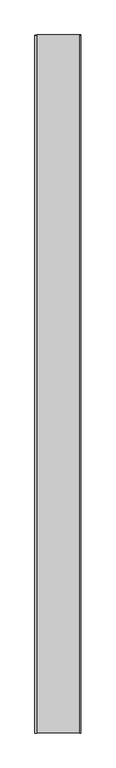
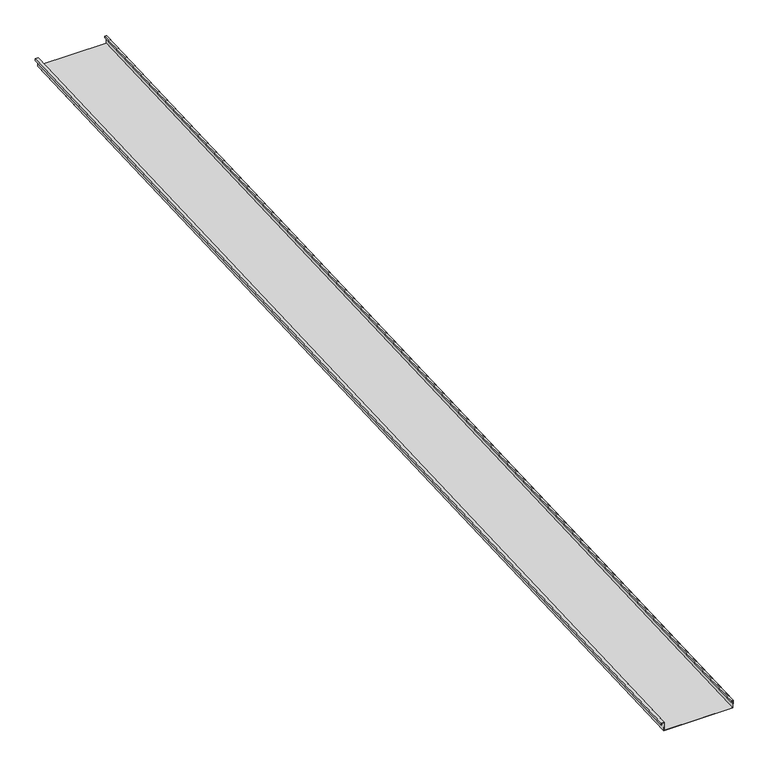
"""IFC4 building model written with IfcOpenShell, lengths in millimetres: proxy geometry, Generic Models 2:Generic Models 2:310765:Generic Models 2:310765 : Generic Models 2:Generic Models 2:310765:103 : Generic Models 2:Generic Models 2:310765:Generic Models 2:310765 : Generic Models 2:Generic Models 2:310765:300385."""

import ifcopenshell
import ifcopenshell.guid

model = None  # the IFC model being written
_history = None  # IfcOwnerHistory: only IFC2X3 demands one
_inside = {}  # id of a spatial element -> (the spatial element, [elements in it])
_under = {}  # id of a project, library or spatial element -> (it, [spatial elements below it])
_declared = {}  # id of a project -> (the project, [libraries it declares])
_typed = {}  # id of a type object -> (the type object, [elements of that type])
_made_of = {}  # id of a material, layer set ... -> (it, [elements and type objects made of it])


def new_model(schema):
    """Start an empty IFC model of exactly this schema.

    Asked for "IFC4X3", IfcOpenShell would pick the latest addendum, in which some entities
    have other attributes; the version numbers below select the first issue.
    IFC2X3 requires an IfcOwnerHistory on every rooted entity: one is made here for all.
    """
    global model, _history
    if schema == "IFC4X3":
        model = ifcopenshell.file(schema_version=(4, 3, 0, 0))
    else:
        model = ifcopenshell.file(schema=schema)
    _inside.clear()
    _under.clear()
    _declared.clear()
    _typed.clear()
    _made_of.clear()
    _history = None
    if model.schema == "IFC2X3":
        org = make("IfcOrganization", Name="unknown")
        user = make(
            "IfcPersonAndOrganization",
            ThePerson=make("IfcPerson", FamilyName="unknown"),
            TheOrganization=org,
        )
        app = make(
            "IfcApplication",
            ApplicationDeveloper=org,
            Version="unknown",
            ApplicationFullName="unknown",
            ApplicationIdentifier="unknown",
        )
        _history = make(
            "IfcOwnerHistory",
            OwningUser=user,
            OwningApplication=app,
            ChangeAction="ADDED",
            CreationDate=0,
        )
    return model


def make(cls, **values):
    """One entity of the class cls with the attributes given. An attribute that is None is left unset."""
    return model.create_entity(
        cls, **{name: value for name, value in values.items() if value is not None}
    )


def rooted(cls, **values):
    """An entity with a GlobalId (a new one), such as an element, a storey or a relation."""
    return make(cls, GlobalId=ifcopenshell.guid.new(), OwnerHistory=_history, **values)


def si_unit(unit_type, name, prefix=None):
    """IfcSIUnit, for example si_unit("LENGTHUNIT", "METRE", prefix="MILLI")."""
    return make("IfcSIUnit", UnitType=unit_type, Prefix=prefix, Name=name)


def assignment(units):
    """IfcUnitAssignment: the units of a project."""
    return None if units is None else make("IfcUnitAssignment", Units=units)


def point(xyz):
    """IfcCartesianPoint."""
    return None if xyz is None else make("IfcCartesianPoint", Coordinates=xyz)


def direction(xyz):
    """IfcDirection."""
    return None if xyz is None else make("IfcDirection", DirectionRatios=xyz)


def frame(location, z_axis=None, x_axis=None):
    """IfcAxis2Placement3D, a coordinate frame: its origin and axes. An axis left out is left unset."""
    return make(
        "IfcAxis2Placement3D",
        Location=point(location),
        Axis=direction(z_axis),
        RefDirection=direction(x_axis),
    )


def origin():
    """The frame at (0, 0, 0) with its axes left unset."""
    return frame((0.0, 0.0, 0.0))


def place(relative_to, where):
    """IfcLocalPlacement: puts the frame where relative to a parent placement (None: the world)."""
    return make(
        "IfcLocalPlacement", PlacementRelTo=relative_to, RelativePlacement=where
    )


def context(
    kind, dimensions, precision=None, world=None, true_north=None, identifier=None
):
    """IfcGeometricRepresentationContext, for example the 3D "Model" context."""
    return make(
        "IfcGeometricRepresentationContext",
        ContextIdentifier=identifier,
        ContextType=kind,
        CoordinateSpaceDimension=dimensions,
        Precision=precision,
        WorldCoordinateSystem=world,
        TrueNorth=true_north,
    )


def project(units=None, contexts=None):
    """IfcProject with its units and contexts."""
    return rooted(
        "IfcProject",
        Name="project",
        RepresentationContexts=contexts,
        UnitsInContext=assignment(units),
    )


def spatial(cls, under=None, at=None, **own):
    """A site, building, storey or space (cls), placed at a placement, below another one or the project."""
    s = rooted(cls, ObjectPlacement=at, **own)
    if under is not None:
        _under.setdefault(under.id(), (under, []))[1].append(s)
    return s


def polyline(points):
    """IfcPolyline through the points."""
    return make("IfcPolyline", Points=[point(p) for p in points])


def outline(outer, holes=None, kind="AREA"):
    """IfcArbitraryClosedProfileDef: a profile drawn as a closed curve; with holes, ...WithVoids."""
    if holes is None:
        return make("IfcArbitraryClosedProfileDef", ProfileType=kind, OuterCurve=outer)
    return make(
        "IfcArbitraryProfileDefWithVoids",
        ProfileType=kind,
        OuterCurve=outer,
        InnerCurves=holes,
    )


def extrude(swept, where, along, depth):
    """IfcExtrudedAreaSolid: the profile swept, set in the frame where, extruded along a direction by depth."""
    return make(
        "IfcExtrudedAreaSolid",
        SweptArea=swept,
        Position=where,
        ExtrudedDirection=direction(along),
        Depth=depth,
    )


def shape(context_of_items, identifier, shape_type, items):
    """IfcShapeRepresentation: the items that make up one representation, for example the "Body"."""
    return make(
        "IfcShapeRepresentation",
        ContextOfItems=context_of_items,
        RepresentationIdentifier=identifier,
        RepresentationType=shape_type,
        Items=items,
    )


def source(mapping_origin, context_of_items, identifier, shape_type, items):
    """IfcRepresentationMap: a shape defined once, which mapped items show again and again."""
    return make(
        "IfcRepresentationMap",
        MappingOrigin=mapping_origin,
        MappedRepresentation=shape(context_of_items, identifier, shape_type, items),
    )


def transform(
    local_origin,
    x_axis=None,
    y_axis=None,
    z_axis=None,
    scale=None,
    scale2=None,
    scale3=None,
    uniform=True,
):
    """IfcCartesianTransformationOperator3D, or its non-uniform kind. x_axis, y_axis, z_axis: its Axis1, 2, 3."""
    if uniform:
        return make(
            "IfcCartesianTransformationOperator3D",
            Axis1=direction(x_axis),
            Axis2=direction(y_axis),
            LocalOrigin=point(local_origin),
            Scale=scale,
            Axis3=direction(z_axis),
        )
    return make(
        "IfcCartesianTransformationOperator3DnonUniform",
        Axis1=direction(x_axis),
        Axis2=direction(y_axis),
        LocalOrigin=point(local_origin),
        Scale=scale,
        Axis3=direction(z_axis),
        Scale2=scale2,
        Scale3=scale3,
    )


def mapped(mapping_source, mapping_target):
    """IfcMappedItem: shows the shape of a source again, moved by a transform."""
    return make(
        "IfcMappedItem", MappingSource=mapping_source, MappingTarget=mapping_target
    )


def made_of(thing, what):
    """Note that an element or type object is made of a material, layer set ...; save() writes the relation."""
    if what is not None:
        _made_of.setdefault(what.id(), (what, []))[1].append(thing)
    return thing


def element(
    cls,
    number,
    at=None,
    inside=None,
    cuts=None,
    type_object=None,
    material=None,
    context=None,
    identifier="Body",
    shape_type=None,
    held_by="IfcProductDefinitionShape",
    body=None,
    shapes=None,
    **own,
):
    """One element of the class cls, such as IfcWall. Its Tag is "e" and its number.

    at: its placement. inside: the storey or other place that contains it. cuts: it is an
    opening in that element (IfcRelVoidsElement). A single representation is given by context,
    identifier, shape_type and body (its items); several are given by shapes. held_by: the class
    of the entity that holds the representations. save() writes the other relations.
    """
    e = rooted(cls, Tag="e%d" % number, ObjectPlacement=at, **own)
    if body is not None:
        shapes = [shape(context, identifier, shape_type, body)]
    if shapes is not None:
        e.Representation = make(held_by, Representations=shapes)
    if inside is not None:
        _inside.setdefault(inside.id(), (inside, []))[1].append(e)
    if cuts is not None:
        rooted(
            "IfcRelVoidsElement", RelatingBuildingElement=cuts, RelatedOpeningElement=e
        )
    if type_object is not None:
        _typed.setdefault(type_object.id(), (type_object, []))[1].append(e)
    return made_of(e, material)


def aggregate(whole, parts):
    """IfcRelAggregates: a whole, such as a stair, and the parts it consists of."""
    return rooted("IfcRelAggregates", RelatingObject=whole, RelatedObjects=parts)


def save(model, path):
    """Write the relations noted so far, then the file.

    IfcRelAggregates (storeys below a building ...), IfcRelContainedInSpatialStructure (elements
    in a storey), IfcRelDefinesByType, IfcRelAssociatesMaterial and IfcRelDeclares: one each for
    every whole, place, type object, material and project.
    """
    for whole, parts in _under.values():
        aggregate(whole, parts)
    for where, things in _inside.values():
        rooted(
            "IfcRelContainedInSpatialStructure",
            RelatedElements=things,
            RelatingStructure=where,
        )
    for kind, things in _typed.values():
        rooted("IfcRelDefinesByType", RelatedObjects=things, RelatingType=kind)
    for what, things in _made_of.values():
        rooted("IfcRelAssociatesMaterial", RelatedObjects=things, RelatingMaterial=what)
    for by, libraries in _declared.values():
        rooted("IfcRelDeclares", RelatingContext=by, RelatedDefinitions=libraries)
    model.write(path)


def generic_models_2d4eb92a(model_context):
    return source(origin(), model_context, "Body", "SweptSolid", [
        extrude(outline(polyline([(1.5875, 0.0), (1.5875, 50.8), (407.9875, 50.8), (407.9875, 1.5875), (396.875, 1.5875), (396.875, 11.1125), (398.4625, 11.1125), (398.4625, 3.175), (406.4, 3.175), (406.4, 49.2125), (3.175, 49.2125), (3.175, -1.5874999), (-14.2875, -1.5874999), (-14.2875, 9.525), (-12.7, 9.525), (-12.7, 0.0), (1.5875, 0.0)])), frame((611102.4263073, -581354.4345603, 3902.6697972), z_axis=(0.0, 0.9991330730923568, 0.041630544712067834), x_axis=(1.0, 0.0, 0.0)), (0.0, 0.0, 1.0), 6400.8),
    ])


if __name__ == "__main__":
    model = new_model("IFC4")
    model_context = context("Model", 3, world=origin())
    ifc_project = project(units=[si_unit("LENGTHUNIT", "METRE", prefix="MILLI")], contexts=[model_context])
    site = spatial("IfcSite", under=ifc_project)
    building = spatial("IfcBuilding", under=site)
    placement = place(None, origin())
    generic_models_shape = generic_models_2d4eb92a(model_context)
    element("IfcBuildingElementProxy", 1, Name="Generic Models 2:Generic Models 2:310765:Generic Models 2:310765 : Generic Models 2:Generic Models 2:310765:103 : Generic Models 2:Generic Models 2:310765:Generic Models 2:310765 : Generic Models 2:Generic Models 2:310765:300385", ObjectType="Generic Models 2:Generic Models 2:310765:Generic Models 2:310765 : Generic Models 2:Generic Models 2:310765:103 : Generic Models 2:Generic Models 2:310765:Generic Models 2:310765 : Generic Models 2:Generic Models 2:310765:300385", at=placement, inside=building, context=model_context, shape_type="MappedRepresentation", body=[
        mapped(generic_models_shape, transform((0.0, 0.0, 0.0), x_axis=(1.0, 0.0, 0.0), y_axis=(0.0, 1.0, 0.0), z_axis=(0.0, 0.0, 1.0))),
    ])
    save(model, "model.ifc")

# Revit data of these elements
# Type "Generic Models 2:Generic Models 2:310765:Generic Models 2:310765 : Generic Models 2:Generic Models 2:310765:103 : Generic Models 2:Generic Models 2:310765:Generic Models 2:310765 : Generic Models 2:Generic Models 2:310765:300385"
#   NameOverride = "Generic Models 2:Generic Models 2:310765:Generic Models 2:310765 : Generic Models 2:Generic Models 2:310765:300385"
#   ObjectTypeOverride = "Generic Models 2:310765 : Generic Models 2:Generic Models 2:310765"
#   Reference = "Generic Models 2"
#   Tag = "300385"
# Element 1 (IfcBuildingElementProxy, "Generic Models 2:Generic Models 2:310765:Generic Models 2:310765 : Generic Models 2:Generic Models 2:310765:103 : Generic Models 2:Generic Models 2:310765:Generic Models 2:310765 : Generic Models 2:Generic Models 2:310765:300385")
#   Materials on its faces: "THERMAL BROKEN ALUMINUM STOREFRONT FOR POLYCARBONATE"
# Materials
#   "THERMAL BROKEN ALUMINUM STOREFRONT FOR POLYCARBONATE": class "Unassigned", colour RGB 244 244 244, transparency 0, Keynote = "M07611300.01", Cost = 0
